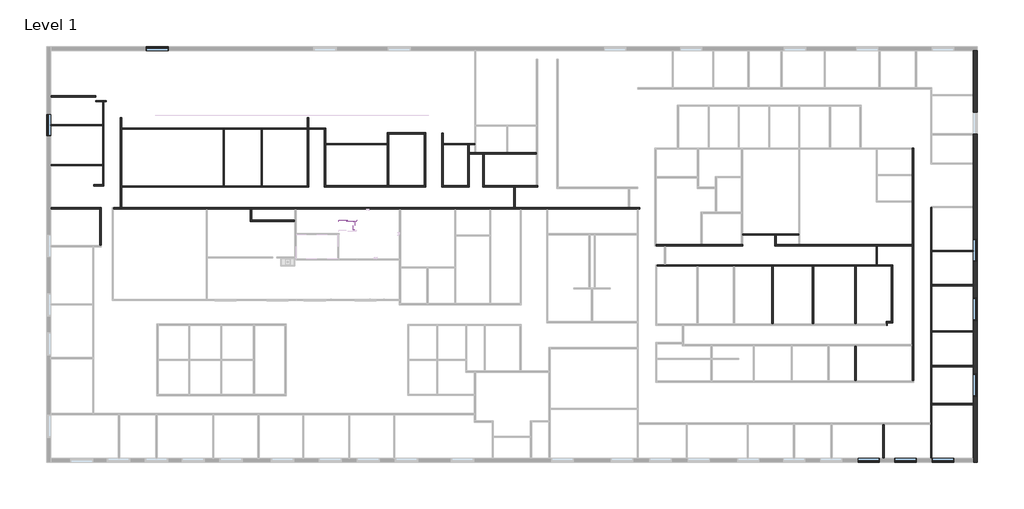
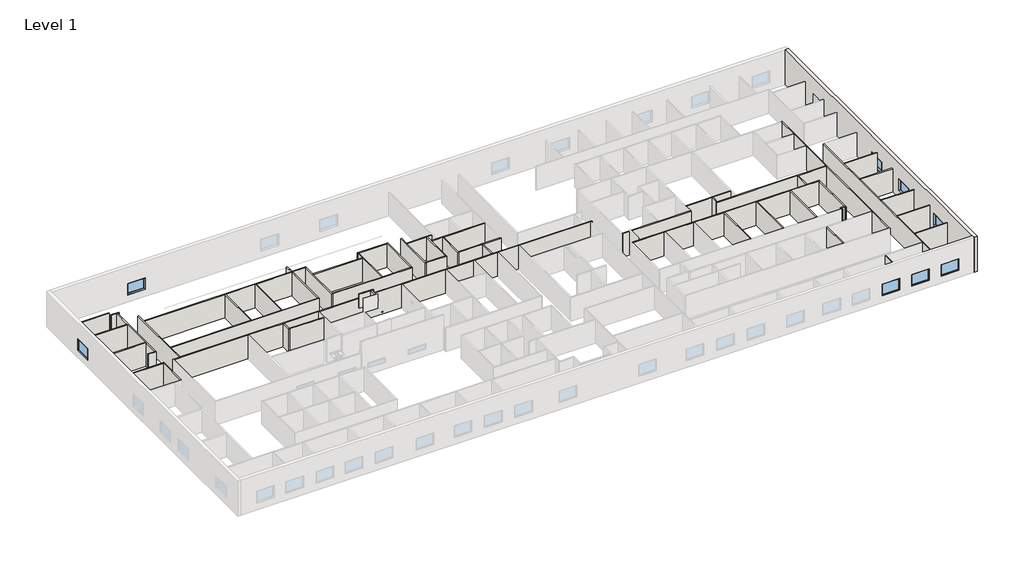
# One storey, part 3 of 4: 55 walls, 8 windows.
# Revit data of these elements (continued)
# Elements 3, 4, 5, 6, 7, 8, 9, 10, 16, 17, 20, 21, 22, 26, 27, 28, 30 (IfcWall, "Interior - 4 7/8\" Partition (1-hr)") (continued)
#   Materials on its faces: "Default Wall", "Gypsum Wall Board"
# Elements 32, 33 (IfcWall, "Interior - 4 7/8\" Partition (1-hr)")
#   built-in parameter 1001111 = 9' - 0"
#   Top Offset = 0' - 0"
#   Base Offset = 9' - 0"
#   Unconnected Height = 6' - 0"
#   wall height = 6' - 0"
#   Phase Created = 03 - Project Completion
#   Base Constraint = Level 1
#   Materials on its faces: "Default Wall", "Gypsum Wall Board"
# Elements 34, 35, 38, 39, 41, 45 (IfcWall, "Interior - 4 7/8\" Partition (1-hr)")
#   Top Offset = 0' - 0"
#   Base Offset = 0' - 0"
#   Unconnected Height = 10' - 0"
#   wall height = 10' - 0"
#   Phase Created = 03 - Project Completion
#   Base Constraint = Level 1
#   Materials on its faces: "Gypsum Wall Board", "Default Wall"
# Elements 36, 37, 40, 42, 43, 44, 46, 47, 48, 49, 50, 51, 52, 53, 54, 55 (IfcWall, "Interior - 4 7/8\" Partition (1-hr)")
#   Top Offset = 0' - 0"
#   Base Offset = 0' - 0"
#   Unconnected Height = 10' - 0"
#   wall height = 10' - 0"
#   Phase Created = 03 - Project Completion
#   Base Constraint = Level 1
#   Materials on its faces: "Default Wall", "Gypsum Wall Board"
# Element 56 (IfcWindow, "Fixed : 86\" x 60\"")
#   Mark = "21"
#   Phase Created = 01 - Existing
#   Materials on its faces: "Sash", "Glass"
# Element 57 (IfcWindow, "Fixed : 86\" x 60\"")
#   Mark = "22"
#   Phase Created = 01 - Existing
#   Materials on its faces: "Sash", "Glass"
# Element 58 (IfcWindow, "Fixed : 86\" x 60\"")
#   Mark = "23"
#   Phase Created = 01 - Existing
#   Materials on its faces: "Sash", "Glass"
# Element 59 (IfcWindow, "Fixed : 86\" x 60\"")
#   Mark = "24"
#   Phase Created = 01 - Existing
#   Materials on its faces: "Sash", "Glass"
# Element 60 (IfcWindow, "Fixed : 86\" x 60\"")
#   Mark = "25"
#   Phase Created = 01 - Existing
#   Materials on its faces: "Sash", "Glass"
# Element 61 (IfcWindow, "Fixed : 86\" x 60\"")
#   Mark = "26"
#   Phase Created = 01 - Existing
#   Materials on its faces: "Sash", "Glass"
# Element 62 (IfcWindow, "Fixed : 86\" x 60\"")
#   Mark = "35"
#   Phase Created = 01 - Existing
#   Materials on its faces: "Sash", "Glass"
# Element 63 (IfcWindow, "Fixed : 86\" x 60\"")
#   Mark = "36"
#   Phase Created = 01 - Existing
#   Materials on its faces: "Sash", "Glass"
# Materials
#   "Metal Stud Layer": class "Metal", colour RGB 199 199 199, transparency 0, Description = "Light gauge steel framing, thermal air layer", Cost = 0
#   "Gypsum Wall Board": class "Generic", colour RGB 127 127 127, transparency 0, Description = "Gypsum Wall Board", Cost = 0
#   "Glass": class "Glass", colour RGB 0 128 192, transparency 0.75, Description = "Soda Lime Glass", Cost = 0
#   "Sash": class "Wood", colour RGB 224 178 126, transparency 0
#   "Default Wall": class "Miscellaneous", colour RGB 128 128 128, transparency 0
